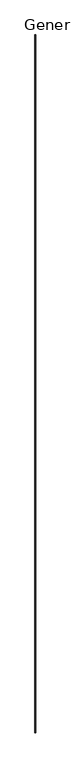
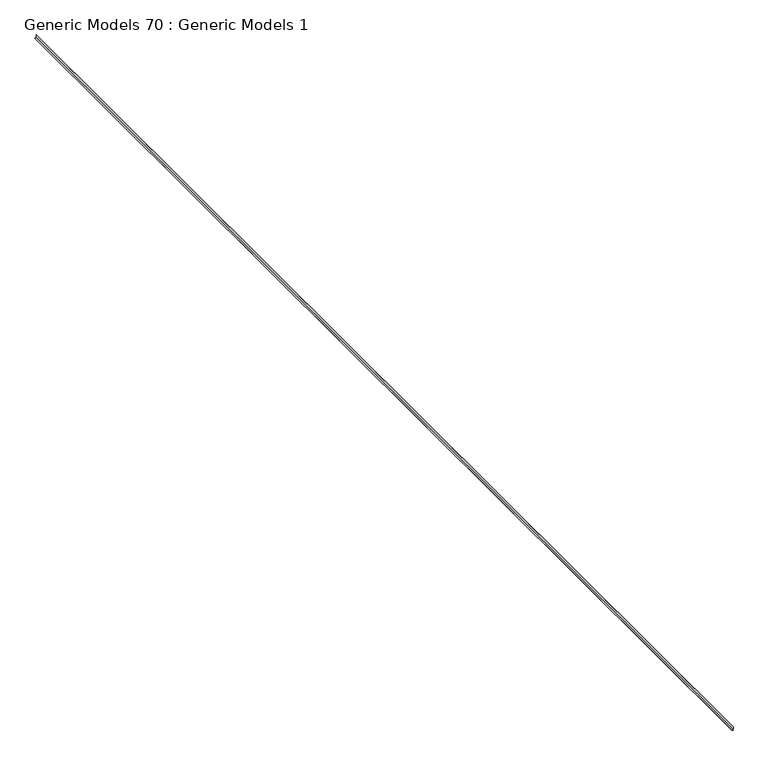
"""IFC4 building model written with IfcOpenShell, lengths in millimetres: proxy geometry, Generic Models 70 : Generic Models 1."""

from ifc_helpers import new_model, si_unit, frame, origin, place, context, project, spatial, polyline, outline, extrude, source, transform, mapped, element, save


def generic_models_70_generic_models_1_b39f0e3d(model_context):
    return source(origin(), model_context, "Body", "SweptSolid", [
        extrude(outline(polyline([(126958.6728942, 8369.1263704), (126952.1949461, 8389.2799869), (126947.8229543, 8390.1033079), (126948.0579859, 8391.3513704), (126953.1727363, 8390.3881753), (126958.6728942, 8373.2765727), (126964.4826506, 8391.3513704), (127009.4728942, 8391.3513704), (127009.4728942, 8390.0813704), (126965.4084299, 8390.0813704), (126958.6728942, 8369.1263704)])), frame((0.0, -7068.1230338, 0.0), z_axis=(0.0, 1.0, 0.0), x_axis=(0.0, 0.0, 1.0)), (0.0, 0.0, 1.0), 19050.0),
    ])


if __name__ == "__main__":
    model = new_model("IFC4")
    model_context = context("Model", 3, world=origin())
    ifc_project = project(units=[si_unit("LENGTHUNIT", "METRE", prefix="MILLI")], contexts=[model_context])
    site = spatial("IfcSite", under=ifc_project)
    building = spatial("IfcBuilding", under=site)
    placement = place(None, origin())
    generic_models_70_generic_models_1_shape = generic_models_70_generic_models_1_b39f0e3d(model_context)
    element("IfcBuildingElementProxy", 1, Name="Generic Models 70 : Generic Models 1", ObjectType="Generic Models 70 : Generic Models 1", at=placement, inside=building, context=model_context, shape_type="MappedRepresentation", body=[
        mapped(generic_models_70_generic_models_1_shape, transform((0.0, 0.0, 0.0), x_axis=(1.0, 0.0, 0.0), y_axis=(0.0, 1.0, 0.0), z_axis=(0.0, 0.0, 1.0))),
    ])
    save(model, "model.ifc")

# Revit data of these elements
# Element 1 (IfcBuildingElementProxy, "Generic Models 70 : Generic Models 1")
#   Materials on its faces: "_16 GA. COPPER WEEP SCREED W/ MIN. 3 1/2\" ATTACHEMENT FLANGE - LAP UNDERLAYMENT OVER WEED SCREED"
# Materials
#   "_16 GA. COPPER WEEP SCREED W/ MIN. 3 1/2\" ATTACHEMENT FLANGE - LAP UNDERLAYMENT OVER WEED SCREED": class "Generic", colour RGB 253 192 103, transparency 0, Cost = 0
